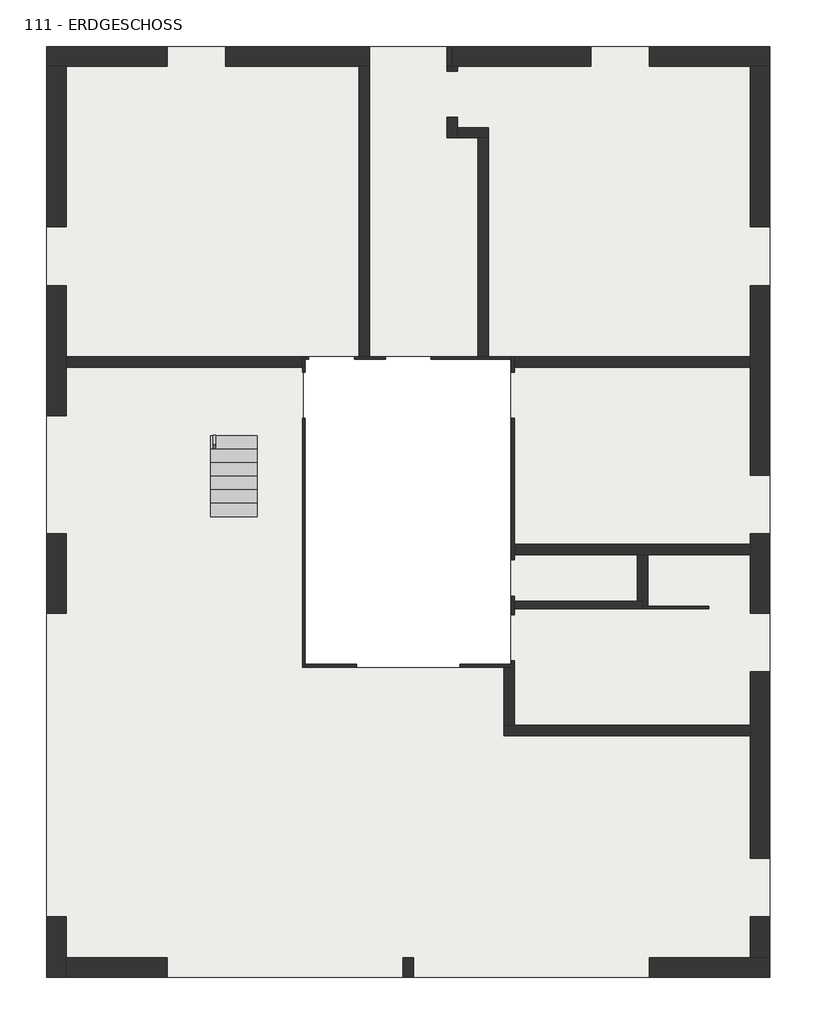
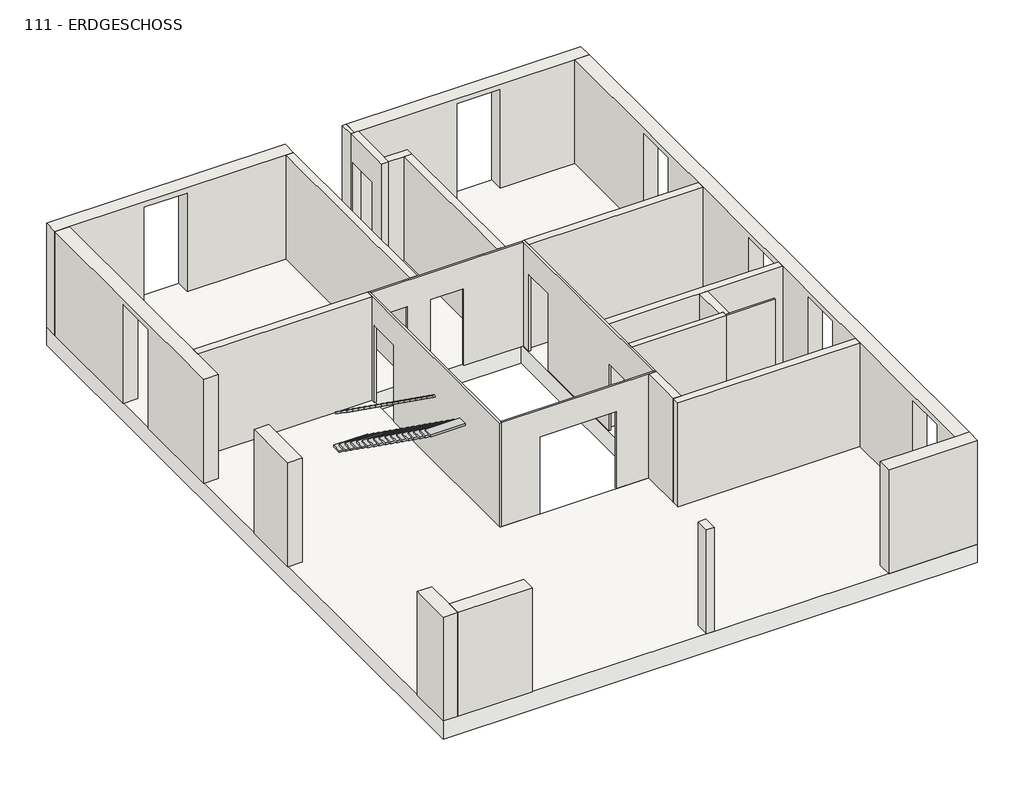
# One storey: 21 walls, 2 stairs, 1 slab.
"""IFC4 building model written with IfcOpenShell, lengths in millimetres."""

import ifcopenshell
import ifcopenshell.guid

model = None  # the IFC model being written
_history = None  # IfcOwnerHistory: only IFC2X3 demands one
_inside = {}  # id of a spatial element -> (the spatial element, [elements in it])
_under = {}  # id of a project, library or spatial element -> (it, [spatial elements below it])
_declared = {}  # id of a project -> (the project, [libraries it declares])
_typed = {}  # id of a type object -> (the type object, [elements of that type])
_made_of = {}  # id of a material, layer set ... -> (it, [elements and type objects made of it])


def new_model(schema):
    """Start an empty IFC model of exactly this schema.

    Asked for "IFC4X3", IfcOpenShell would pick the latest addendum, in which some entities
    have other attributes; the version numbers below select the first issue.
    IFC2X3 requires an IfcOwnerHistory on every rooted entity: one is made here for all.
    """
    global model, _history
    if schema == "IFC4X3":
        model = ifcopenshell.file(schema_version=(4, 3, 0, 0))
    else:
        model = ifcopenshell.file(schema=schema)
    _inside.clear()
    _under.clear()
    _declared.clear()
    _typed.clear()
    _made_of.clear()
    _history = None
    if model.schema == "IFC2X3":
        org = make("IfcOrganization", Name="unknown")
        user = make(
            "IfcPersonAndOrganization",
            ThePerson=make("IfcPerson", FamilyName="unknown"),
            TheOrganization=org,
        )
        app = make(
            "IfcApplication",
            ApplicationDeveloper=org,
            Version="unknown",
            ApplicationFullName="unknown",
            ApplicationIdentifier="unknown",
        )
        _history = make(
            "IfcOwnerHistory",
            OwningUser=user,
            OwningApplication=app,
            ChangeAction="ADDED",
            CreationDate=0,
        )
    return model


def make(cls, **values):
    """One entity of the class cls with the attributes given. An attribute that is None is left unset."""
    return model.create_entity(
        cls, **{name: value for name, value in values.items() if value is not None}
    )


def rooted(cls, **values):
    """An entity with a GlobalId (a new one), such as an element, a storey or a relation."""
    return make(cls, GlobalId=ifcopenshell.guid.new(), OwnerHistory=_history, **values)


def si_unit(unit_type, name, prefix=None):
    """IfcSIUnit, for example si_unit("LENGTHUNIT", "METRE", prefix="MILLI")."""
    return make("IfcSIUnit", UnitType=unit_type, Prefix=prefix, Name=name)


def assignment(units):
    """IfcUnitAssignment: the units of a project."""
    return None if units is None else make("IfcUnitAssignment", Units=units)


def point(xyz):
    """IfcCartesianPoint."""
    return None if xyz is None else make("IfcCartesianPoint", Coordinates=xyz)


def direction(xyz):
    """IfcDirection."""
    return None if xyz is None else make("IfcDirection", DirectionRatios=xyz)


def frame(location, z_axis=None, x_axis=None):
    """IfcAxis2Placement3D, a coordinate frame: its origin and axes. An axis left out is left unset."""
    return make(
        "IfcAxis2Placement3D",
        Location=point(location),
        Axis=direction(z_axis),
        RefDirection=direction(x_axis),
    )


def origin():
    """The frame at (0, 0, 0) with its axes left unset."""
    return frame((0.0, 0.0, 0.0))


def origin_with_axes():
    """The frame at (0, 0, 0) with the z axis (0, 0, 1) and the x axis (1, 0, 0) written out."""
    return frame((0.0, 0.0, 0.0), z_axis=(0.0, 0.0, 1.0), x_axis=(1.0, 0.0, 0.0))


def place(relative_to, where):
    """IfcLocalPlacement: puts the frame where relative to a parent placement (None: the world)."""
    return make(
        "IfcLocalPlacement", PlacementRelTo=relative_to, RelativePlacement=where
    )


def context(
    kind, dimensions, precision=None, world=None, true_north=None, identifier=None
):
    """IfcGeometricRepresentationContext, for example the 3D "Model" context."""
    return make(
        "IfcGeometricRepresentationContext",
        ContextIdentifier=identifier,
        ContextType=kind,
        CoordinateSpaceDimension=dimensions,
        Precision=precision,
        WorldCoordinateSystem=world,
        TrueNorth=true_north,
    )


def project(units=None, contexts=None):
    """IfcProject with its units and contexts."""
    return rooted(
        "IfcProject",
        Name="project",
        RepresentationContexts=contexts,
        UnitsInContext=assignment(units),
    )


def spatial(cls, under=None, at=None, **own):
    """A site, building, storey or space (cls), placed at a placement, below another one or the project."""
    s = rooted(cls, ObjectPlacement=at, **own)
    if under is not None:
        _under.setdefault(under.id(), (under, []))[1].append(s)
    return s


def polyline(points):
    """IfcPolyline through the points."""
    return make("IfcPolyline", Points=[point(p) for p in points])


def outline(outer, holes=None, kind="AREA"):
    """IfcArbitraryClosedProfileDef: a profile drawn as a closed curve; with holes, ...WithVoids."""
    if holes is None:
        return make("IfcArbitraryClosedProfileDef", ProfileType=kind, OuterCurve=outer)
    return make(
        "IfcArbitraryProfileDefWithVoids",
        ProfileType=kind,
        OuterCurve=outer,
        InnerCurves=holes,
    )


def extrude(swept, where, along, depth):
    """IfcExtrudedAreaSolid: the profile swept, set in the frame where, extruded along a direction by depth."""
    return make(
        "IfcExtrudedAreaSolid",
        SweptArea=swept,
        Position=where,
        ExtrudedDirection=direction(along),
        Depth=depth,
    )


def faces_of(points, faces, orient=None, outer=None):
    """IfcFace entities. A face is a list of loops; a loop is a list of indices into points, from 0.

    orient and outer hold one flag for each loop. By default every Orientation is true, the
    first loop of a face is its IfcFaceOuterBound and the others are IfcFaceBound.
    """
    made = []
    for i, loops in enumerate(faces):
        bounds = []
        for j, loop in enumerate(loops):
            is_outer = j == 0 if outer is None else outer[i][j]
            bounds.append(
                make(
                    "IfcFaceOuterBound" if is_outer else "IfcFaceBound",
                    Bound=make("IfcPolyLoop", Polygon=[points[k] for k in loop]),
                    Orientation=True if orient is None else orient[i][j],
                )
            )
        made.append(make("IfcFace", Bounds=bounds))
    return made


def faceted_brep(points, faces, orient=None, outer=None, voids=None):
    """IfcFacetedBrep: a solid bounded by flat faces; with voids (closed shells), ...WithVoids."""
    shared = [point(p) for p in points]
    hull = make("IfcClosedShell", CfsFaces=faces_of(shared, faces, orient, outer))
    if voids is None:
        return make("IfcFacetedBrep", Outer=hull)
    return make(
        "IfcFacetedBrepWithVoids",
        Outer=hull,
        Voids=[
            make(cls, CfsFaces=faces_of(shared, fs, o, b)) for cls, fs, o, b in voids
        ],
    )


def shape(context_of_items, identifier, shape_type, items):
    """IfcShapeRepresentation: the items that make up one representation, for example the "Body"."""
    return make(
        "IfcShapeRepresentation",
        ContextOfItems=context_of_items,
        RepresentationIdentifier=identifier,
        RepresentationType=shape_type,
        Items=items,
    )


def source(mapping_origin, context_of_items, identifier, shape_type, items):
    """IfcRepresentationMap: a shape defined once, which mapped items show again and again."""
    return make(
        "IfcRepresentationMap",
        MappingOrigin=mapping_origin,
        MappedRepresentation=shape(context_of_items, identifier, shape_type, items),
    )


def transform(
    local_origin,
    x_axis=None,
    y_axis=None,
    z_axis=None,
    scale=None,
    scale2=None,
    scale3=None,
    uniform=True,
):
    """IfcCartesianTransformationOperator3D, or its non-uniform kind. x_axis, y_axis, z_axis: its Axis1, 2, 3."""
    if uniform:
        return make(
            "IfcCartesianTransformationOperator3D",
            Axis1=direction(x_axis),
            Axis2=direction(y_axis),
            LocalOrigin=point(local_origin),
            Scale=scale,
            Axis3=direction(z_axis),
        )
    return make(
        "IfcCartesianTransformationOperator3DnonUniform",
        Axis1=direction(x_axis),
        Axis2=direction(y_axis),
        LocalOrigin=point(local_origin),
        Scale=scale,
        Axis3=direction(z_axis),
        Scale2=scale2,
        Scale3=scale3,
    )


def mapped(mapping_source, mapping_target):
    """IfcMappedItem: shows the shape of a source again, moved by a transform."""
    return make(
        "IfcMappedItem", MappingSource=mapping_source, MappingTarget=mapping_target
    )


def made_of(thing, what):
    """Note that an element or type object is made of a material, layer set ...; save() writes the relation."""
    if what is not None:
        _made_of.setdefault(what.id(), (what, []))[1].append(thing)
    return thing


def element(
    cls,
    number,
    at=None,
    inside=None,
    cuts=None,
    type_object=None,
    material=None,
    context=None,
    identifier="Body",
    shape_type=None,
    held_by="IfcProductDefinitionShape",
    body=None,
    shapes=None,
    **own,
):
    """One element of the class cls, such as IfcWall. Its Tag is "e" and its number.

    at: its placement. inside: the storey or other place that contains it. cuts: it is an
    opening in that element (IfcRelVoidsElement). A single representation is given by context,
    identifier, shape_type and body (its items); several are given by shapes. held_by: the class
    of the entity that holds the representations. save() writes the other relations.
    """
    e = rooted(cls, Tag="e%d" % number, ObjectPlacement=at, **own)
    if body is not None:
        shapes = [shape(context, identifier, shape_type, body)]
    if shapes is not None:
        e.Representation = make(held_by, Representations=shapes)
    if inside is not None:
        _inside.setdefault(inside.id(), (inside, []))[1].append(e)
    if cuts is not None:
        rooted(
            "IfcRelVoidsElement", RelatingBuildingElement=cuts, RelatedOpeningElement=e
        )
    if type_object is not None:
        _typed.setdefault(type_object.id(), (type_object, []))[1].append(e)
    return made_of(e, material)


def aggregate(whole, parts):
    """IfcRelAggregates: a whole, such as a stair, and the parts it consists of."""
    return rooted("IfcRelAggregates", RelatingObject=whole, RelatedObjects=parts)


def save(model, path):
    """Write the relations noted so far, then the file.

    IfcRelAggregates (storeys below a building ...), IfcRelContainedInSpatialStructure (elements
    in a storey), IfcRelDefinesByType, IfcRelAssociatesMaterial and IfcRelDeclares: one each for
    every whole, place, type object, material and project.
    """
    for whole, parts in _under.values():
        aggregate(whole, parts)
    for where, things in _inside.values():
        rooted(
            "IfcRelContainedInSpatialStructure",
            RelatedElements=things,
            RelatingStructure=where,
        )
    for kind, things in _typed.values():
        rooted("IfcRelDefinesByType", RelatedObjects=things, RelatingType=kind)
    for what, things in _made_of.values():
        rooted("IfcRelAssociatesMaterial", RelatedObjects=things, RelatingMaterial=what)
    for by, libraries in _declared.values():
        rooted("IfcRelDeclares", RelatingContext=by, RelatedDefinitions=libraries)
    model.write(path)


def slab_87d51967(model_context):
    return source(origin(), model_context, "Body", "SweptSolid", [
        extrude(outline(polyline([(15500.0, 1547.1380981), (1500.0, 1547.1380981), (1500.0, 19550.0), (15500.0, 19550.0), (15500.0, 1547.1380981)]), holes=[polyline([(10475.0, 13550.0), (6475.0, 13550.0), (6475.0, 7550.0), (10475.0, 7550.0), (10475.0, 13550.0)])]), frame((0.0, 0.0, -500.0), z_axis=(0.0, 0.0, 1.0), x_axis=(1.0, 0.0, 0.0)), (0.0, 0.0, 1.0), 500.0),
    ])


def stair_a78379cc(model_context):
    return source(origin(), model_context, "Body", "SweptSolid", [
        extrude(outline(polyline([(0.0, -319.1002977), (0.0, 0.0), (50.0, 0.0), (50.0, -319.1002977), (0.0, -319.1002977)])), frame((162072.7593015, 34520.3024209, 4178.947508), z_axis=(0.0, 0.5797550216229128, 0.8147908411997622), x_axis=(-1.0, 0.0, 0.0)), (0.0, 0.0, 1.0), 50.0),
        extrude(outline(polyline([(0.0, -319.1002977), (0.0, 0.0), (50.0, 0.0), (50.0, -319.1002977), (0.0, -319.1002977)])), frame((162072.7593015, 34780.3024209, 3993.947508), z_axis=(0.0, 0.5797550216228999, 0.8147908411997712), x_axis=(-1.0, 0.0, 0.0)), (0.0, 0.0, 1.0), 50.0),
        extrude(outline(polyline([(0.0, -319.1002977), (0.0, 0.0), (50.0, 0.0), (50.0, -319.1002977), (0.0, -319.1002977)])), frame((162072.7593015, 35040.3024209, 3808.947508), z_axis=(0.0, 0.5797550216229128, 0.8147908411997622), x_axis=(-1.0, 0.0, 0.0)), (0.0, 0.0, 1.0), 50.0),
        extrude(outline(polyline([(0.0, -319.1002977), (0.0, 0.0), (50.0, 0.0), (50.0, -319.1002977), (0.0, -319.1002977)])), frame((162072.7593015, 35300.3024209, 3623.947508), z_axis=(0.0, 0.5797550216229086, 0.8147908411997651), x_axis=(-1.0, 0.0, 0.0)), (0.0, 0.0, 1.0), 50.0),
        extrude(outline(polyline([(0.0, -319.1002977), (0.0, 0.0), (50.0, 0.0), (50.0, -319.1002977), (0.0, -319.1002977)])), frame((162072.7593015, 35560.3024209, 3438.947508), z_axis=(0.0, 0.5797550216229094, 0.8147908411997645), x_axis=(-1.0, 0.0, 0.0)), (0.0, 0.0, 1.0), 50.0),
        extrude(outline(polyline([(0.0, -319.1002977), (0.0, 0.0), (50.0, 0.0), (50.0, -319.1002977), (0.0, -319.1002977)])), frame((162072.7593015, 35820.3024209, 3253.947508), z_axis=(0.0, 0.5797550216229012, 0.8147908411997705), x_axis=(-1.0, 0.0, 0.0)), (0.0, 0.0, 1.0), 50.0),
        extrude(outline(polyline([(0.0, -319.1002977), (0.0, 0.0), (50.0, 0.0), (50.0, -319.1002977), (0.0, -319.1002977)])), frame((162072.7593015, 36080.3024209, 3068.947508), z_axis=(0.0, 0.5797550216229139, 0.8147908411997614), x_axis=(-1.0, 0.0, 0.0)), (0.0, 0.0, 1.0), 50.0),
        extrude(outline(polyline([(0.0, -319.1002977), (0.0, 0.0), (50.0, 0.0), (50.0, -319.1002977), (0.0, -319.1002977)])), frame((162072.7593015, 36340.3024209, 2883.947508), z_axis=(0.0, 0.579755021622915, 0.8147908411997605), x_axis=(-1.0, 0.0, 0.0)), (0.0, 0.0, 1.0), 50.0),
        extrude(outline(polyline([(0.0, -319.1002977), (0.0, 0.0), (50.0, 0.0), (50.0, -319.1002977), (0.0, -319.1002977)])), frame((162072.7593015, 36600.3024209, 2698.947508), z_axis=(0.0, 0.5797550216229116, 0.814790841199763), x_axis=(-1.0, 0.0, 0.0)), (0.0, 0.0, 1.0), 50.0),
        extrude(outline(polyline([(0.0, -319.1002977), (0.0, 0.0), (50.0, 0.0), (50.0, -319.1002977), (0.0, -319.1002977)])), frame((162072.7593015, 36860.3024209, 2513.947508), z_axis=(0.0, 0.5797550216228977, 0.8147908411997729), x_axis=(-1.0, 0.0, 0.0)), (0.0, 0.0, 1.0), 50.0),
        extrude(outline(polyline([(0.0, -319.1002977), (0.0, 0.0), (50.0, 0.0), (50.0, -319.1002977), (0.0, -319.1002977)])), frame((162072.7593015, 37120.3024209, 2328.947508), z_axis=(0.0, 0.5797550216229123, 0.8147908411997625), x_axis=(-1.0, 0.0, 0.0)), (0.0, 0.0, 1.0), 50.0),
        extrude(outline(polyline([(0.0, -319.1002977), (0.0, 0.0), (50.0, 0.0), (50.0, -319.1002977), (0.0, -319.1002977)])), frame((162072.7593015, 37380.3024209, 2143.947508), z_axis=(0.0, 0.5797550216229145, 0.814790841199761), x_axis=(-1.0, 0.0, 0.0)), (0.0, 0.0, 1.0), 50.0),
        extrude(outline(polyline([(0.0, -319.1002977), (0.0, 0.0), (50.0, 0.0), (50.0, -319.1002977), (0.0, -319.1002977)])), frame((162072.7593015, 37640.3024209, 1958.947508), z_axis=(0.0, 0.5797550216228994, 0.8147908411997717), x_axis=(-1.0, 0.0, 0.0)), (0.0, 0.0, 1.0), 50.0),
        extrude(outline(polyline([(0.0, -319.1002977), (0.0, 0.0), (50.0, 0.0), (50.0, -319.1002977), (0.0, -319.1002977)])), frame((162072.7593015, 37900.3024209, 1773.947508), z_axis=(0.0, 0.579755021622915, 0.8147908411997605), x_axis=(-1.0, 0.0, 0.0)), (0.0, 0.0, 1.0), 50.0),
        extrude(outline(polyline([(0.0, -319.1002977), (0.0, 0.0), (50.0, 0.0), (50.0, -319.1002977), (0.0, -319.1002977)])), frame((162072.7593015, 38160.3024209, 1588.947508), z_axis=(0.0, 0.5797550216229086, 0.8147908411997651), x_axis=(-1.0, 0.0, 0.0)), (0.0, 0.0, 1.0), 50.0),
        extrude(outline(polyline([(0.0, -319.1002977), (0.0, 0.0), (50.0, 0.0), (50.0, -319.1002977), (0.0, -319.1002977)])), frame((162072.7593015, 38420.3024209, 1403.947508), z_axis=(0.0, 0.5797550216229066, 0.8147908411997665), x_axis=(-1.0, 0.0, 0.0)), (0.0, 0.0, 1.0), 50.0),
        extrude(outline(polyline([(0.0, -319.1002977), (0.0, 0.0), (50.0, 0.0), (50.0, -319.1002977), (0.0, -319.1002977)])), frame((162072.7593015, 38680.3024209, 1218.947508), z_axis=(0.0, 0.5797550216228988, 0.8147908411997722), x_axis=(-1.0, 0.0, 0.0)), (0.0, 0.0, 1.0), 50.0),
        extrude(outline(polyline([(161972.7593015, 38694.7962965), (161972.7593015, 38954.7962965), (162872.7593015, 38954.7962965), (162872.7593015, 38694.7962965), (161972.7593015, 38694.7962965)])), frame((0.0, 0.0, 135.0), z_axis=(0.0, 0.0, 1.0), x_axis=(1.0, 0.0, 0.0)), (0.0, 0.0, 1.0), 50.0),
        extrude(outline(polyline([(161972.7593015, 38434.7962965), (161972.7593015, 38694.7962965), (162872.7593015, 38694.7962965), (162872.7593015, 38434.7962965), (161972.7593015, 38434.7962965)])), frame((0.0, 0.0, 320.0), z_axis=(0.0, 0.0, 1.0), x_axis=(1.0, 0.0, 0.0)), (0.0, 0.0, 1.0), 50.0),
        extrude(outline(polyline([(161972.7593015, 38174.7962965), (161972.7593015, 38434.7962965), (162872.7593015, 38434.7962965), (162872.7593015, 38174.7962965), (161972.7593015, 38174.7962965)])), frame((0.0, 0.0, 505.0), z_axis=(0.0, 0.0, 1.0), x_axis=(1.0, 0.0, 0.0)), (0.0, 0.0, 1.0), 50.0),
        extrude(outline(polyline([(161972.7593015, 37914.7962965), (161972.7593015, 38174.7962965), (162872.7593015, 38174.7962965), (162872.7593015, 37914.7962965), (161972.7593015, 37914.7962965)])), frame((0.0, 0.0, 690.0), z_axis=(0.0, 0.0, 1.0), x_axis=(1.0, 0.0, 0.0)), (0.0, 0.0, 1.0), 50.0),
        extrude(outline(polyline([(161972.7593015, 37654.7962965), (161972.7593015, 37914.7962965), (162872.7593015, 37914.7962965), (162872.7593015, 37654.7962965), (161972.7593015, 37654.7962965)])), frame((0.0, 0.0, 875.0), z_axis=(0.0, 0.0, 1.0), x_axis=(1.0, 0.0, 0.0)), (0.0, 0.0, 1.0), 50.0),
        extrude(outline(polyline([(161972.7593015, 37394.7962965), (161972.7593015, 37654.7962965), (162872.7593015, 37654.7962965), (162872.7593015, 37394.7962965), (161972.7593015, 37394.7962965)])), frame((0.0, 0.0, 1060.0), z_axis=(0.0, 0.0, 1.0), x_axis=(1.0, 0.0, 0.0)), (0.0, 0.0, 1.0), 50.0),
        extrude(outline(polyline([(161972.7593015, 37134.7962965), (161972.7593015, 37394.7962965), (162872.7593015, 37394.7962965), (162872.7593015, 37134.7962965), (161972.7593015, 37134.7962965)])), frame((0.0, 0.0, 1245.0), z_axis=(0.0, 0.0, 1.0), x_axis=(1.0, 0.0, 0.0)), (0.0, 0.0, 1.0), 50.0),
        extrude(outline(polyline([(161972.7593015, 36874.7962965), (161972.7593015, 37134.7962965), (162872.7593015, 37134.7962965), (162872.7593015, 36874.7962965), (161972.7593015, 36874.7962965)])), frame((0.0, 0.0, 1430.0), z_axis=(0.0, 0.0, 1.0), x_axis=(1.0, 0.0, 0.0)), (0.0, 0.0, 1.0), 50.0),
        extrude(outline(polyline([(161972.7593015, 36614.7962965), (161972.7593015, 36874.7962965), (162872.7593015, 36874.7962965), (162872.7593015, 36614.7962965), (161972.7593015, 36614.7962965)])), frame((0.0, 0.0, 1615.0), z_axis=(0.0, 0.0, 1.0), x_axis=(1.0, 0.0, 0.0)), (0.0, 0.0, 1.0), 50.0),
        extrude(outline(polyline([(161972.7593015, 36354.7962965), (161972.7593015, 36614.7962965), (162872.7593015, 36614.7962965), (162872.7593015, 36354.7962965), (161972.7593015, 36354.7962965)])), frame((0.0, 0.0, 1800.0), z_axis=(0.0, 0.0, 1.0), x_axis=(1.0, 0.0, 0.0)), (0.0, 0.0, 1.0), 50.0),
        extrude(outline(polyline([(161972.7593015, 36094.7962965), (161972.7593015, 36354.7962965), (162872.7593015, 36354.7962965), (162872.7593015, 36094.7962965), (161972.7593015, 36094.7962965)])), frame((0.0, 0.0, 1985.0), z_axis=(0.0, 0.0, 1.0), x_axis=(1.0, 0.0, 0.0)), (0.0, 0.0, 1.0), 50.0),
        extrude(outline(polyline([(161972.7593015, 35834.7962965), (161972.7593015, 36094.7962965), (162872.7593015, 36094.7962965), (162872.7593015, 35834.7962965), (161972.7593015, 35834.7962965)])), frame((0.0, 0.0, 2170.0), z_axis=(0.0, 0.0, 1.0), x_axis=(1.0, 0.0, 0.0)), (0.0, 0.0, 1.0), 50.0),
        extrude(outline(polyline([(161972.7593015, 35574.7962965), (161972.7593015, 35834.7962965), (162872.7593015, 35834.7962965), (162872.7593015, 35574.7962965), (161972.7593015, 35574.7962965)])), frame((0.0, 0.0, 2355.0), z_axis=(0.0, 0.0, 1.0), x_axis=(1.0, 0.0, 0.0)), (0.0, 0.0, 1.0), 50.0),
        extrude(outline(polyline([(161972.7593015, 35314.7962965), (161972.7593015, 35574.7962965), (162872.7593015, 35574.7962965), (162872.7593015, 35314.7962965), (161972.7593015, 35314.7962965)])), frame((0.0, 0.0, 2540.0), z_axis=(0.0, 0.0, 1.0), x_axis=(1.0, 0.0, 0.0)), (0.0, 0.0, 1.0), 50.0),
        extrude(outline(polyline([(161972.7593015, 35054.7962965), (161972.7593015, 35314.7962965), (162872.7593015, 35314.7962965), (162872.7593015, 35054.7962965), (161972.7593015, 35054.7962965)])), frame((0.0, 0.0, 2725.0), z_axis=(0.0, 0.0, 1.0), x_axis=(1.0, 0.0, 0.0)), (0.0, 0.0, 1.0), 50.0),
        extrude(outline(polyline([(161972.7593015, 34794.7962965), (161972.7593015, 35054.7962965), (162872.7593015, 35054.7962965), (162872.7593015, 34794.7962965), (161972.7593015, 34794.7962965)])), frame((0.0, 0.0, 2910.0), z_axis=(0.0, 0.0, 1.0), x_axis=(1.0, 0.0, 0.0)), (0.0, 0.0, 1.0), 50.0),
        extrude(outline(polyline([(161972.7593015, 34534.7962965), (161972.7593015, 34794.7962965), (162872.7593015, 34794.7962965), (162872.7593015, 34534.7962965), (161972.7593015, 34534.7962965)])), frame((0.0, 0.0, 3095.0), z_axis=(0.0, 0.0, 1.0), x_axis=(1.0, 0.0, 0.0)), (0.0, 0.0, 1.0), 50.0),
    ])


def stair_667f7fc2(model_context):
    return source(origin(), model_context, "Body", "SweptSolid", [
        extrude(outline(polyline([(0.0, -319.1002977), (0.0, 0.0), (50.0, 0.0), (50.0, -319.1002977), (0.0, -319.1002977)])), frame((162072.7593015, 34520.3024209, 4178.947508), z_axis=(0.0, 0.5797550216229128, 0.8147908411997622), x_axis=(-1.0, 0.0, 0.0)), (0.0, 0.0, 1.0), 50.0),
        extrude(outline(polyline([(0.0, -319.1002977), (0.0, 0.0), (50.0, 0.0), (50.0, -319.1002977), (0.0, -319.1002977)])), frame((162072.7593015, 34780.3024209, 3993.947508), z_axis=(0.0, 0.5797550216229022, 0.8147908411997696), x_axis=(-1.0, 0.0, 0.0)), (0.0, 0.0, 1.0), 50.0),
        extrude(outline(polyline([(0.0, -319.1002977), (0.0, 0.0), (50.0, 0.0), (50.0, -319.1002977), (0.0, -319.1002977)])), frame((162072.7593015, 35040.3024209, 3808.947508), z_axis=(0.0, 0.5797550216229116, 0.814790841199763), x_axis=(-1.0, 0.0, 0.0)), (0.0, 0.0, 1.0), 50.0),
        extrude(outline(polyline([(0.0, -319.1002977), (0.0, 0.0), (50.0, 0.0), (50.0, -319.1002977), (0.0, -319.1002977)])), frame((162072.7593015, 35300.3024209, 3623.947508), z_axis=(0.0, 0.5797550216229086, 0.8147908411997651), x_axis=(-1.0, 0.0, 0.0)), (0.0, 0.0, 1.0), 50.0),
        extrude(outline(polyline([(0.0, -319.1002977), (0.0, 0.0), (50.0, 0.0), (50.0, -319.1002977), (0.0, -319.1002977)])), frame((162072.7593015, 35560.3024209, 3438.947508), z_axis=(0.0, 0.5797550216229094, 0.8147908411997645), x_axis=(-1.0, 0.0, 0.0)), (0.0, 0.0, 1.0), 50.0),
        extrude(outline(polyline([(0.0, -319.1002977), (0.0, 0.0), (50.0, 0.0), (50.0, -319.1002977), (0.0, -319.1002977)])), frame((162072.7593015, 35820.3024209, 3253.947508), z_axis=(0.0, 0.5797550216228999, 0.8147908411997712), x_axis=(-1.0, 0.0, 0.0)), (0.0, 0.0, 1.0), 50.0),
        extrude(outline(polyline([(0.0, -319.1002977), (0.0, 0.0), (50.0, 0.0), (50.0, -319.1002977), (0.0, -319.1002977)])), frame((162072.7593015, 36080.3024209, 3068.947508), z_axis=(0.0, 0.579755021622915, 0.8147908411997605), x_axis=(-1.0, 0.0, 0.0)), (0.0, 0.0, 1.0), 50.0),
        extrude(outline(polyline([(0.0, -319.1002977), (0.0, 0.0), (50.0, 0.0), (50.0, -319.1002977), (0.0, -319.1002977)])), frame((162072.7593015, 36340.3024209, 2883.947508), z_axis=(0.0, 0.5797550216229139, 0.8147908411997614), x_axis=(-1.0, 0.0, 0.0)), (0.0, 0.0, 1.0), 50.0),
        extrude(outline(polyline([(0.0, -319.1002977), (0.0, 0.0), (50.0, 0.0), (50.0, -319.1002977), (0.0, -319.1002977)])), frame((162072.7593015, 36600.3024209, 2698.947508), z_axis=(0.0, 0.5797550216229128, 0.8147908411997622), x_axis=(-1.0, 0.0, 0.0)), (0.0, 0.0, 1.0), 50.0),
        extrude(outline(polyline([(0.0, -319.1002977), (0.0, 0.0), (50.0, 0.0), (50.0, -319.1002977), (0.0, -319.1002977)])), frame((162072.7593015, 36860.3024209, 2513.947508), z_axis=(0.0, 0.5797550216228966, 0.8147908411997736), x_axis=(-1.0, 0.0, 0.0)), (0.0, 0.0, 1.0), 50.0),
        extrude(outline(polyline([(0.0, -319.1002977), (0.0, 0.0), (50.0, 0.0), (50.0, -319.1002977), (0.0, -319.1002977)])), frame((162072.7593015, 37120.3024209, 2328.947508), z_axis=(0.0, 0.5797550216229123, 0.8147908411997625), x_axis=(-1.0, 0.0, 0.0)), (0.0, 0.0, 1.0), 50.0),
        extrude(outline(polyline([(0.0, -319.1002977), (0.0, 0.0), (50.0, 0.0), (50.0, -319.1002977), (0.0, -319.1002977)])), frame((162072.7593015, 37380.3024209, 2143.947508), z_axis=(0.0, 0.5797550216229139, 0.8147908411997614), x_axis=(-1.0, 0.0, 0.0)), (0.0, 0.0, 1.0), 50.0),
        extrude(outline(polyline([(0.0, -319.1002977), (0.0, 0.0), (50.0, 0.0), (50.0, -319.1002977), (0.0, -319.1002977)])), frame((162072.7593015, 37640.3024209, 1958.947508), z_axis=(0.0, 0.5797550216228999, 0.8147908411997712), x_axis=(-1.0, 0.0, 0.0)), (0.0, 0.0, 1.0), 50.0),
        extrude(outline(polyline([(0.0, -319.1002977), (0.0, 0.0), (50.0, 0.0), (50.0, -319.1002977), (0.0, -319.1002977)])), frame((162072.7593015, 37900.3024209, 1773.947508), z_axis=(0.0, 0.579755021622915, 0.8147908411997605), x_axis=(-1.0, 0.0, 0.0)), (0.0, 0.0, 1.0), 50.0),
        extrude(outline(polyline([(0.0, -319.1002977), (0.0, 0.0), (50.0, 0.0), (50.0, -319.1002977), (0.0, -319.1002977)])), frame((162072.7593015, 38160.3024209, 1588.947508), z_axis=(0.0, 0.579755021622908, 0.8147908411997654), x_axis=(-1.0, 0.0, 0.0)), (0.0, 0.0, 1.0), 50.0),
        extrude(outline(polyline([(0.0, -319.1002977), (0.0, 0.0), (50.0, 0.0), (50.0, -319.1002977), (0.0, -319.1002977)])), frame((162072.7593015, 38420.3024209, 1403.947508), z_axis=(0.0, 0.5797550216229066, 0.8147908411997665), x_axis=(-1.0, 0.0, 0.0)), (0.0, 0.0, 1.0), 50.0),
        extrude(outline(polyline([(0.0, -319.1002977), (0.0, 0.0), (50.0, 0.0), (50.0, -319.1002977), (0.0, -319.1002977)])), frame((162072.7593015, 38680.3024209, 1218.947508), z_axis=(0.0, 0.5797550216228985, 0.8147908411997723), x_axis=(-1.0, 0.0, 0.0)), (0.0, 0.0, 1.0), 50.0),
        extrude(outline(polyline([(161972.7593015, 38694.7962965), (161972.7593015, 38954.7962965), (162872.7593015, 38954.7962965), (162872.7593015, 38694.7962965), (161972.7593015, 38694.7962965)])), frame((0.0, 0.0, 135.0), z_axis=(0.0, 0.0, 1.0), x_axis=(1.0, 0.0, 0.0)), (0.0, 0.0, 1.0), 50.0),
        extrude(outline(polyline([(161972.7593015, 38434.7962965), (161972.7593015, 38694.7962965), (162872.7593015, 38694.7962965), (162872.7593015, 38434.7962965), (161972.7593015, 38434.7962965)])), frame((0.0, 0.0, 320.0), z_axis=(0.0, 0.0, 1.0), x_axis=(1.0, 0.0, 0.0)), (0.0, 0.0, 1.0), 50.0),
        extrude(outline(polyline([(161972.7593015, 38174.7962965), (161972.7593015, 38434.7962965), (162872.7593015, 38434.7962965), (162872.7593015, 38174.7962965), (161972.7593015, 38174.7962965)])), frame((0.0, 0.0, 505.0), z_axis=(0.0, 0.0, 1.0), x_axis=(1.0, 0.0, 0.0)), (0.0, 0.0, 1.0), 50.0),
        extrude(outline(polyline([(161972.7593015, 37914.7962965), (161972.7593015, 38174.7962965), (162872.7593015, 38174.7962965), (162872.7593015, 37914.7962965), (161972.7593015, 37914.7962965)])), frame((0.0, 0.0, 690.0), z_axis=(0.0, 0.0, 1.0), x_axis=(1.0, 0.0, 0.0)), (0.0, 0.0, 1.0), 50.0),
        extrude(outline(polyline([(161972.7593015, 37654.7962965), (161972.7593015, 37914.7962965), (162872.7593015, 37914.7962965), (162872.7593015, 37654.7962965), (161972.7593015, 37654.7962965)])), frame((0.0, 0.0, 875.0), z_axis=(0.0, 0.0, 1.0), x_axis=(1.0, 0.0, 0.0)), (0.0, 0.0, 1.0), 50.0),
        extrude(outline(polyline([(161972.7593015, 37394.7962965), (161972.7593015, 37654.7962965), (162872.7593015, 37654.7962965), (162872.7593015, 37394.7962965), (161972.7593015, 37394.7962965)])), frame((0.0, 0.0, 1060.0), z_axis=(0.0, 0.0, 1.0), x_axis=(1.0, 0.0, 0.0)), (0.0, 0.0, 1.0), 50.0),
        extrude(outline(polyline([(161972.7593015, 37134.7962965), (161972.7593015, 37394.7962965), (162872.7593015, 37394.7962965), (162872.7593015, 37134.7962965), (161972.7593015, 37134.7962965)])), frame((0.0, 0.0, 1245.0), z_axis=(0.0, 0.0, 1.0), x_axis=(1.0, 0.0, 0.0)), (0.0, 0.0, 1.0), 50.0),
        extrude(outline(polyline([(161972.7593015, 36874.7962965), (161972.7593015, 37134.7962965), (162872.7593015, 37134.7962965), (162872.7593015, 36874.7962965), (161972.7593015, 36874.7962965)])), frame((0.0, 0.0, 1430.0), z_axis=(0.0, 0.0, 1.0), x_axis=(1.0, 0.0, 0.0)), (0.0, 0.0, 1.0), 50.0),
        extrude(outline(polyline([(161972.7593015, 36614.7962965), (161972.7593015, 36874.7962965), (162872.7593015, 36874.7962965), (162872.7593015, 36614.7962965), (161972.7593015, 36614.7962965)])), frame((0.0, 0.0, 1615.0), z_axis=(0.0, 0.0, 1.0), x_axis=(1.0, 0.0, 0.0)), (0.0, 0.0, 1.0), 50.0),
        extrude(outline(polyline([(161972.7593015, 36354.7962965), (161972.7593015, 36614.7962965), (162872.7593015, 36614.7962965), (162872.7593015, 36354.7962965), (161972.7593015, 36354.7962965)])), frame((0.0, 0.0, 1800.0), z_axis=(0.0, 0.0, 1.0), x_axis=(1.0, 0.0, 0.0)), (0.0, 0.0, 1.0), 50.0),
        extrude(outline(polyline([(161972.7593015, 36094.7962965), (161972.7593015, 36354.7962965), (162872.7593015, 36354.7962965), (162872.7593015, 36094.7962965), (161972.7593015, 36094.7962965)])), frame((0.0, 0.0, 1985.0), z_axis=(0.0, 0.0, 1.0), x_axis=(1.0, 0.0, 0.0)), (0.0, 0.0, 1.0), 50.0),
        extrude(outline(polyline([(161972.7593015, 35834.7962965), (161972.7593015, 36094.7962965), (162872.7593015, 36094.7962965), (162872.7593015, 35834.7962965), (161972.7593015, 35834.7962965)])), frame((0.0, 0.0, 2170.0), z_axis=(0.0, 0.0, 1.0), x_axis=(1.0, 0.0, 0.0)), (0.0, 0.0, 1.0), 50.0),
        extrude(outline(polyline([(161972.7593015, 35574.7962965), (161972.7593015, 35834.7962965), (162872.7593015, 35834.7962965), (162872.7593015, 35574.7962965), (161972.7593015, 35574.7962965)])), frame((0.0, 0.0, 2355.0), z_axis=(0.0, 0.0, 1.0), x_axis=(1.0, 0.0, 0.0)), (0.0, 0.0, 1.0), 50.0),
        extrude(outline(polyline([(161972.7593015, 35314.7962965), (161972.7593015, 35574.7962965), (162872.7593015, 35574.7962965), (162872.7593015, 35314.7962965), (161972.7593015, 35314.7962965)])), frame((0.0, 0.0, 2540.0), z_axis=(0.0, 0.0, 1.0), x_axis=(1.0, 0.0, 0.0)), (0.0, 0.0, 1.0), 50.0),
        extrude(outline(polyline([(161972.7593015, 35054.7962965), (161972.7593015, 35314.7962965), (162872.7593015, 35314.7962965), (162872.7593015, 35054.7962965), (161972.7593015, 35054.7962965)])), frame((0.0, 0.0, 2725.0), z_axis=(0.0, 0.0, 1.0), x_axis=(1.0, 0.0, 0.0)), (0.0, 0.0, 1.0), 50.0),
        extrude(outline(polyline([(161972.7593015, 34794.7962965), (161972.7593015, 35054.7962965), (162872.7593015, 35054.7962965), (162872.7593015, 34794.7962965), (161972.7593015, 34794.7962965)])), frame((0.0, 0.0, 2910.0), z_axis=(0.0, 0.0, 1.0), x_axis=(1.0, 0.0, 0.0)), (0.0, 0.0, 1.0), 50.0),
        extrude(outline(polyline([(161972.7593015, 34534.7962965), (161972.7593015, 34794.7962965), (162872.7593015, 34794.7962965), (162872.7593015, 34534.7962965), (161972.7593015, 34534.7962965)])), frame((0.0, 0.0, 3095.0), z_axis=(0.0, 0.0, 1.0), x_axis=(1.0, 0.0, 0.0)), (0.0, 0.0, 1.0), 50.0),
    ])


model = new_model("IFC4")

# Units and contexts
model_context = context("Model", 3, world=origin())
ifc_project = project(units=[si_unit("LENGTHUNIT", "METRE", prefix="MILLI")], contexts=[model_context])

# Site, building, storey
site = spatial("IfcSite", under=ifc_project)
building = spatial("IfcBuilding", under=site)
storey = spatial("IfcBuildingStorey", under=building, Name="111 - ERDGESCHOSS", Elevation=0.0)

# Slab
placement = place(None, origin())
slab_shape = slab_87d51967(model_context)
element("IfcSlab", 1, ObjectType="Holzdecke : Holzdecke", at=placement, inside=storey, context=model_context, shape_type="MappedRepresentation", body=[
    mapped(slab_shape, transform((0.0, 0.0, 0.0), x_axis=(1.0, 0.0, 0.0), y_axis=(0.0, 1.0, 0.0), z_axis=(0.0, 0.0, 1.0))),
])

# Stairs
stair_shape = stair_a78379cc(model_context)
element("IfcStair", 2, ObjectType="  :  ", at=placement, inside=storey, context=model_context, shape_type="MappedRepresentation", body=[
    mapped(stair_shape, transform((-157297.7593015, -26934.7962965, 0.0), x_axis=(1.0, 0.0, 0.0), y_axis=(0.0, 1.0, 0.0), z_axis=(0.0, 0.0, 1.0))),
])
stair_2_shape = stair_667f7fc2(model_context)
element("IfcStair", 3, ObjectType="  92587 :   92587", at=placement, inside=storey, context=model_context, shape_type="MappedRepresentation", body=[
    mapped(stair_2_shape, transform((-157297.7593015, -26934.7962965, 0.0), x_axis=(1.0, 0.0, 0.0), y_axis=(0.0, 1.0, 0.0), z_axis=(0.0, 0.0, 1.0))),
])

# Walls
element("IfcWall", 4, ObjectType="Holzwand:1129", at=placement, inside=storey, context=model_context, shape_type="SweptSolid", body=[
    extrude(outline(polyline([(7750.0, 19170.0), (7750.0, 13550.0), (7550.0, 13550.0), (7550.0, 19170.0), (7750.0, 19170.0)])), origin_with_axes(), (0.0, 0.0, 1.0), 2880.0),
])
element("IfcWall", 5, ObjectType="Holzwand:1130", at=placement, inside=storey, context=model_context, shape_type="SweptSolid", body=[
    extrude(outline(polyline([(6450.0, 13350.0), (1880.0, 13350.0), (1880.0, 13550.0), (6450.0, 13550.0), (6450.0, 13350.0)])), origin_with_axes(), (0.0, 0.0, 1.0), 2880.0),
])
element("IfcWall", 6, ObjectType="Holzwand:1131", at=placement, inside=storey, context=model_context, shape_type="Brep", body=[
    faceted_brep([(10050.0, 17981.8742346, 0.0), (9450.0, 17981.8742346, 0.0), (9450.0, 17981.8742346, 2880.0), (10050.0, 17981.8742346, 2880.0), (10050.0, 17781.8742346, 0.0), (10050.0, 17781.8742346, 2880.0), (9850.0, 17781.8742346, 2880.0), (9450.0, 17781.8742346, 2880.0), (9450.0, 17781.8742346, 0.0), (9850.0, 17781.8742346, 0.0)], [[[0, 1, 2, 3]], [[4, 5, 6, 7, 8, 9]], [[1, 0, 4, 9, 8]], [[3, 2, 7, 6, 5]], [[0, 3, 5, 4]], [[2, 1, 8, 7]]]),
])
element("IfcWall", 7, ObjectType="Holzwand:1132", at=placement, inside=storey, context=model_context, shape_type="Brep", body=[
    faceted_brep([(9450.0, 19170.0, 2880.0), (9450.0, 17981.8742346, 2880.0), (9450.0, 17781.8742346, 2880.0), (9450.0, 17781.8742346, 0.0), (9450.0, 17981.8742346, 0.0), (9450.0, 18184.2114284, 0.0), (9450.0, 18184.2114284, 2135.0), (9450.0, 19069.2114284, 2135.0), (9450.0, 19069.2114284, 0.0), (9450.0, 19170.0, 0.0), (9250.0, 17781.8742346, 2880.0), (9250.0, 19170.0, 2880.0), (9250.0, 19170.0, 0.0), (9250.0, 19069.2114284, 0.0), (9250.0, 19069.2114284, 2135.0), (9250.0, 18184.2114284, 2135.0), (9250.0, 18184.2114284, 0.0), (9250.0, 17781.8742346, 0.0)], [[[0, 1, 2, 3, 4, 5, 6, 7, 8, 9]], [[10, 11, 12, 13, 14, 15, 16, 17]], [[3, 17, 16, 5, 4]], [[12, 9, 8, 13]], [[2, 1, 0, 11, 10]], [[15, 6, 5, 16]], [[6, 15, 14, 7]], [[7, 14, 13, 8]], [[3, 2, 10, 17]], [[0, 9, 12, 11]]]),
])
element("IfcWall", 8, ObjectType="Holzwand:1133", at=placement, inside=storey, context=model_context, shape_type="SweptSolid", body=[
    extrude(outline(polyline([(10050.0, 17781.8742346), (10050.0, 13550.0), (9850.0, 13550.0), (9850.0, 17781.8742346), (10050.0, 17781.8742346)])), origin_with_axes(), (0.0, 0.0, 1.0), 2880.0),
])
element("IfcWall", 9, ObjectType="Holzwand:1134", at=placement, inside=storey, context=model_context, shape_type="SweptSolid", body=[
    extrude(outline(polyline([(15120.0, 13350.0), (10550.0, 13350.0), (10550.0, 13550.0), (15120.0, 13550.0), (15120.0, 13350.0)])), origin_with_axes(), (0.0, 0.0, 1.0), 2880.0),
])
element("IfcWall", 10, ObjectType="Holzwand:1136", at=placement, inside=storey, context=model_context, shape_type="Brep", body=[
    faceted_brep([(15120.0, 6425.0, 0.0), (10550.0, 6425.0, 0.0), (10350.0, 6425.0, 0.0), (10350.0, 6425.0, 2880.0), (10550.0, 6425.0, 2880.0), (15120.0, 6425.0, 2880.0), (15120.0, 6225.0, 0.0), (15120.0, 6225.0, 2880.0), (10350.0, 6225.0, 2880.0), (10350.0, 6225.0, 0.0)], [[[0, 1, 2, 3, 4, 5]], [[6, 7, 8, 9]], [[2, 1, 0, 6, 9]], [[5, 4, 3, 8, 7]], [[0, 5, 7, 6]], [[3, 2, 9, 8]]]),
])
element("IfcWall", 11, ObjectType="Holzwand:1137", at=placement, inside=storey, context=model_context, shape_type="SweptSolid", body=[
    extrude(outline(polyline([(10550.0, 9925.0), (15120.0, 9925.0), (15120.0, 9725.0), (10550.0, 9725.0), (10550.0, 9925.0)])), origin_with_axes(), (0.0, 0.0, 1.0), 2880.0),
])
element("IfcWall", 12, ObjectType="Holzwand:1139", at=placement, inside=storey, context=model_context, shape_type="SweptSolid", body=[
    extrude(outline(polyline([(10350.0, 6425.0), (10350.0, 7550.0), (10550.0, 7550.0), (10550.0, 6425.0), (10350.0, 6425.0)])), origin_with_axes(), (0.0, 0.0, 1.0), 2880.0),
])
element("IfcWall", 13, ObjectType="Holzwand:1143", at=placement, inside=storey, context=model_context, shape_type="Brep", body=[
    faceted_brep([(13035.0, 8825.0, 0.0), (12935.0, 8825.0, 0.0), (10550.0, 8825.0, 0.0), (10550.0, 8825.0, 2880.0), (12935.0, 8825.0, 2880.0), (13035.0, 8825.0, 2880.0), (13035.0, 8675.0, 0.0), (13035.0, 8675.0, 2880.0), (10550.0, 8675.0, 2880.0), (10550.0, 8675.0, 0.0), (13035.0, 8725.0, 0.0), (13035.0, 8725.0, 2880.0)], [[[0, 1, 2, 3, 4, 5]], [[6, 7, 8, 9]], [[2, 1, 0, 10, 6, 9]], [[3, 2, 9, 8]], [[5, 4, 3, 8, 7, 11]], [[0, 5, 11, 7, 6, 10]]]),
])
element("IfcWall", 14, ObjectType="Holzwand:1144", at=placement, inside=storey, context=model_context, shape_type="Brep", body=[
    faceted_brep([(13035.0, 8675.0, 0.0), (14320.0, 8675.0, 0.0), (14320.0, 8675.0, 2880.0), (13035.0, 8675.0, 2880.0), (13035.0, 8725.0, 0.0), (13035.0, 8725.0, 2880.0), (13135.0, 8725.0, 2880.0), (14320.0, 8725.0, 2880.0), (14320.0, 8725.0, 0.0), (13135.0, 8725.0, 0.0)], [[[0, 1, 2, 3]], [[4, 5, 6, 7, 8, 9]], [[1, 0, 4, 9, 8]], [[2, 1, 8, 7]], [[3, 2, 7, 6, 5]], [[0, 3, 5, 4]]]),
])
element("IfcWall", 15, ObjectType="Holzwand:1145", at=placement, inside=storey, context=model_context, shape_type="SweptSolid", body=[
    extrude(outline(polyline([(12935.0, 8825.0), (12935.0, 9725.0), (13135.0, 9725.0), (13135.0, 8725.0), (13035.0, 8725.0), (13035.0, 8825.0), (12935.0, 8825.0)])), origin_with_axes(), (0.0, 0.0, 1.0), 2880.0),
])
element("IfcWall", 16, ObjectType=" :1146", at=placement, inside=storey, context=model_context, shape_type="Brep", body=[
    faceted_brep([(6500.0, 13550.0, 2880.0), (6500.0, 13500.0, 2880.0), (6500.0, 7600.0, 2880.0), (6500.0, 7550.0, 2880.0), (6500.0, 7550.0, 0.0), (6500.0, 7600.0, 0.0), (6500.0, 12363.6489699, 0.0), (6500.0, 12363.6489699, 2135.0), (6500.0, 13248.6489699, 2135.0), (6500.0, 13248.6489699, 0.0), (6500.0, 13500.0, 0.0), (6500.0, 13550.0, 0.0), (6450.0, 7550.0, 2880.0), (6450.0, 13550.0, 2880.0), (6450.0, 13550.0, 0.0), (6450.0, 13248.6489699, 0.0), (6450.0, 13248.6489699, 2135.0), (6450.0, 12363.6489699, 2135.0), (6450.0, 12363.6489699, 0.0), (6450.0, 7550.0, 0.0)], [[[0, 1, 2, 3, 4, 5, 6, 7, 8, 9, 10, 11]], [[12, 13, 14, 15, 16, 17, 18, 19]], [[14, 11, 10, 9, 15]], [[4, 19, 18, 6, 5]], [[3, 2, 1, 0, 13, 12]], [[8, 16, 15, 9]], [[16, 8, 7, 17]], [[17, 7, 6, 18]], [[0, 11, 14, 13]], [[4, 3, 12, 19]]]),
])
element("IfcWall", 17, ObjectType=" :1147", at=placement, inside=storey, context=model_context, shape_type="SweptSolid", body=[
    extrude(outline(polyline([(2880.0, 10500.0), (2880.0, 6500.0), (0.0, 6500.0), (0.0, 6572.8375746), (2150.0, 6572.8375746), (2150.0, 7457.8375746), (0.0, 7457.8375746), (0.0, 8057.5), (2135.0, 8057.5), (2135.0, 8942.5), (0.0, 8942.5), (0.0, 10500.0), (2880.0, 10500.0)])), frame((0.0, 13500.0, 0.0), z_axis=(0.0, 1.0, 0.0), x_axis=(0.0, 0.0, 1.0)), (0.0, 0.0, 1.0), 50.0),
])
element("IfcWall", 18, ObjectType=" :1148", at=placement, inside=storey, context=model_context, shape_type="Brep", body=[
    faceted_brep([(6500.0, 7600.0, 2880.0), (10500.0, 7600.0, 2880.0), (10550.0, 7600.0, 2880.0), (10550.0, 7600.0, 0.0), (10500.0, 7600.0, 0.0), (9500.0, 7600.0, 0.0), (9500.0, 7600.0, 2135.0), (7500.0, 7600.0, 2135.0), (7500.0, 7600.0, 0.0), (6500.0, 7600.0, 0.0), (10550.0, 7550.0, 2880.0), (6500.0, 7550.0, 2880.0), (6500.0, 7550.0, 0.0), (7500.0, 7550.0, 0.0), (7500.0, 7550.0, 2135.0), (9500.0, 7550.0, 2135.0), (9500.0, 7550.0, 0.0), (10550.0, 7550.0, 0.0)], [[[0, 1, 2, 3, 4, 5, 6, 7, 8, 9]], [[10, 11, 12, 13, 14, 15, 16, 17]], [[3, 17, 16, 5, 4]], [[12, 9, 8, 13]], [[2, 1, 0, 11, 10]], [[7, 14, 13, 8]], [[14, 7, 6, 15]], [[15, 6, 5, 16]], [[3, 2, 10, 17]], [[0, 9, 12, 11]]]),
])
element("IfcWall", 19, ObjectType=" :1149", at=placement, inside=storey, context=model_context, shape_type="Brep", body=[
    faceted_brep([(10500.0, 7600.0, 2880.0), (10500.0, 13500.0, 2880.0), (10500.0, 13550.0, 2880.0), (10500.0, 13550.0, 0.0), (10500.0, 13500.0, 0.0), (10500.0, 13248.6489699, 0.0), (10500.0, 13248.6489699, 2135.0), (10500.0, 12363.6489699, 2135.0), (10500.0, 12363.6489699, 0.0), (10500.0, 9621.2509729, 0.0), (10500.0, 9621.2509729, 1860.0), (10500.0, 8921.2509729, 1860.0), (10500.0, 8921.2509729, 0.0), (10500.0, 8561.3454038, 0.0), (10500.0, 8561.3454038, 1860.0), (10500.0, 7676.3454038, 1860.0), (10500.0, 7676.3454038, 0.0), (10500.0, 7600.0, 0.0), (10550.0, 13550.0, 2880.0), (10550.0, 7600.0, 2880.0), (10550.0, 7600.0, 0.0), (10550.0, 7676.3454038, 0.0), (10550.0, 7676.3454038, 1860.0), (10550.0, 8561.3454038, 1860.0), (10550.0, 8561.3454038, 0.0), (10550.0, 8921.2509729, 0.0), (10550.0, 8921.2509729, 1860.0), (10550.0, 9621.2509729, 1860.0), (10550.0, 9621.2509729, 0.0), (10550.0, 12363.6489699, 0.0), (10550.0, 12363.6489699, 2135.0), (10550.0, 13248.6489699, 2135.0), (10550.0, 13248.6489699, 0.0), (10550.0, 13550.0, 0.0)], [[[0, 1, 2, 3, 4, 5, 6, 7, 8, 9, 10, 11, 12, 13, 14, 15, 16, 17]], [[18, 19, 20, 21, 22, 23, 24, 25, 26, 27, 28, 29, 30, 31, 32, 33]], [[12, 25, 24, 13]], [[28, 9, 8, 29]], [[17, 16, 21, 20]], [[3, 33, 32, 5, 4]], [[2, 1, 0, 19, 18]], [[11, 26, 25, 12]], [[26, 11, 10, 27]], [[27, 10, 9, 28]], [[23, 14, 13, 24]], [[14, 23, 22, 15]], [[15, 22, 21, 16]], [[7, 30, 29, 8]], [[30, 7, 6, 31]], [[31, 6, 5, 32]], [[3, 2, 18, 33]], [[0, 17, 20, 19]]]),
])
element("IfcWall", 20, ObjectType="1141 Aussenwand", at=placement, inside=storey, context=model_context, shape_type="Brep", body=[
    faceted_brep([(1880.0, 10124.602585, 0.0), (1880.0, 10124.602585, 2880.0), (1880.0, 8593.5588642, 2880.0), (1880.0, 8593.5588642, 0.0), (1500.0, 10124.602585, 2880.0), (1500.0, 10124.602585, 0.0), (1500.0, 8593.5588642, 0.0), (1500.0, 8593.5588642, 2880.0)], [[[0, 1, 2, 3]], [[4, 5, 6, 7]], [[5, 0, 3, 6]], [[1, 4, 7, 2]], [[1, 0, 5, 4]], [[3, 2, 7, 6]]]),
    faceted_brep([(1880.0, 19170.0, 2880.0), (1880.0, 12409.602585, 2880.0), (1880.0, 12409.602585, 0.0), (1880.0, 14926.9335014, 0.0), (1880.0, 14926.9335014, 2740.0), (1880.0, 16061.9335014, 2740.0), (1880.0, 16061.9335014, 0.0), (1880.0, 19170.0, 0.0), (1500.0, 12409.602585, 2880.0), (1500.0, 19170.0, 2880.0), (1500.0, 19170.0, 0.0), (1500.0, 16061.9335014, 0.0), (1500.0, 16061.9335014, 2740.0), (1500.0, 14926.9335014, 2740.0), (1500.0, 14926.9335014, 0.0), (1500.0, 12409.602585, 0.0)], [[[0, 1, 2, 3, 4, 5, 6, 7]], [[8, 9, 10, 11, 12, 13, 14, 15]], [[2, 15, 14, 3]], [[7, 6, 11, 10]], [[1, 0, 9, 8]], [[2, 1, 8, 15]], [[5, 12, 11, 6]], [[12, 5, 4, 13]], [[13, 4, 3, 14]], [[0, 7, 10, 9]]]),
    faceted_brep([(1880.0, 1547.1380981, 0.0), (1880.0, 1927.1380981, 0.0), (1880.0, 2716.7406831, 0.0), (1880.0, 2716.7406831, 2880.0), (1880.0, 1927.1380981, 2880.0), (1880.0, 1547.1380981, 2880.0), (1500.0, 1547.1380981, 2880.0), (1500.0, 2716.7406831, 2880.0), (1500.0, 2716.7406831, 0.0), (1500.0, 1547.1380981, 0.0)], [[[0, 1, 2, 3, 4, 5]], [[6, 7, 8, 9]], [[2, 1, 0, 9, 8]], [[5, 4, 3, 7, 6]], [[3, 2, 8, 7]], [[0, 5, 6, 9]]]),
])
element("IfcWall", 21, ObjectType="1141 Aussenwand", at=placement, inside=storey, context=model_context, shape_type="SweptSolid", body=[
    extrude(outline(polyline([(1927.1380981, 2880.0), (19170.0, 2880.0), (19170.0, 0.0), (16061.9335014, 0.0), (16061.9335014, 2740.0), (14926.9335014, 2740.0), (14926.9335014, 0.0), (11259.602585, 0.0), (11259.602585, 2740.0), (10124.602585, 2740.0), (10124.602585, 0.0), (8593.5588642, 0.0), (8593.5588642, 2740.0), (7458.5588642, 2740.0), (7458.5588642, 0.0), (3852.1380981, 0.0), (3852.1380981, 2740.0), (2717.1380981, 2740.0), (2717.1380981, 0.0), (1927.1380981, 0.0), (1927.1380981, 2880.0)])), frame((15120.0, 0.0, 0.0), z_axis=(1.0, 0.0, 0.0), x_axis=(0.0, 1.0, 0.0)), (0.0, 0.0, 1.0), 380.0),
])
element("IfcWall", 22, ObjectType="1141 Aussenwand", at=placement, inside=storey, context=model_context, shape_type="Brep", body=[
    faceted_brep([(8600.0, 1927.1380981, 2880.0), (8600.0, 1927.1380981, 0.0), (8399.2893219, 1927.1380981, 0.0), (8399.2893219, 1927.1380981, 2880.0), (8600.0, 1547.1380981, 0.0), (8600.0, 1547.1380981, 2880.0), (8399.2893219, 1547.1380981, 2880.0), (8399.2893219, 1547.1380981, 0.0)], [[[0, 1, 2, 3]], [[4, 5, 6, 7]], [[1, 4, 7, 2]], [[5, 0, 3, 6]], [[1, 0, 5, 4]], [[3, 2, 7, 6]]]),
    faceted_brep([(1880.0, 1927.1380981, 2880.0), (3830.0, 1927.1380981, 2880.0), (3830.0, 1927.1380981, 0.0), (1880.0, 1927.1380981, 0.0), (1880.0, 1547.1380981, 0.0), (3830.0, 1547.1380981, 0.0), (3830.0, 1547.1380981, 2880.0), (1880.0, 1547.1380981, 2880.0)], [[[0, 1, 2, 3]], [[4, 5, 6, 7]], [[3, 2, 5, 4]], [[1, 0, 7, 6]], [[2, 1, 6, 5]], [[0, 3, 4, 7]]]),
    faceted_brep([(15500.0, 1927.1380981, 0.0), (15120.0, 1927.1380981, 0.0), (13170.0, 1927.1380981, 0.0), (13170.0, 1927.1380981, 2880.0), (15120.0, 1927.1380981, 2880.0), (15500.0, 1927.1380981, 2880.0), (15500.0, 1547.1380981, 2880.0), (13170.0, 1547.1380981, 2880.0), (13170.0, 1547.1380981, 0.0), (15500.0, 1547.1380981, 0.0)], [[[0, 1, 2, 3, 4, 5]], [[6, 7, 8, 9]], [[2, 1, 0, 9, 8]], [[5, 4, 3, 7, 6]], [[3, 2, 8, 7]], [[0, 5, 6, 9]]]),
])
element("IfcWall", 23, ObjectType="1141 Aussenwand", at=placement, inside=storey, context=model_context, shape_type="Brep", body=[
    faceted_brep([(1500.0, 19170.0, 0.0), (1880.0, 19170.0, 0.0), (3830.0, 19170.0, 0.0), (3830.0, 19170.0, 2740.0), (4965.0, 19170.0, 2740.0), (4965.0, 19170.0, 0.0), (7750.0, 19170.0, 0.0), (7750.0, 19170.0, 2880.0), (1880.0, 19170.0, 2880.0), (1500.0, 19170.0, 2880.0), (3830.0, 19550.0, 0.0), (1500.0, 19550.0, 0.0), (1500.0, 19550.0, 2880.0), (7750.0, 19550.0, 2880.0), (7750.0, 19550.0, 0.0), (4965.0, 19550.0, 0.0), (4965.0, 19550.0, 2740.0), (3830.0, 19550.0, 2740.0)], [[[0, 1, 2, 3, 4, 5, 6, 7, 8, 9]], [[10, 11, 12, 13, 14, 15, 16, 17]], [[5, 15, 14, 6]], [[2, 1, 0, 11, 10]], [[12, 9, 8, 7, 13]], [[17, 3, 2, 10]], [[3, 17, 16, 4]], [[4, 16, 15, 5]], [[7, 6, 14, 13]], [[0, 9, 12, 11]]]),
    faceted_brep([(9350.0, 19170.0, 0.0), (9350.0, 19170.0, 2880.0), (9250.0, 19170.0, 2880.0), (9250.0, 19170.0, 0.0), (9350.0, 19550.0, 2880.0), (9350.0, 19550.0, 0.0), (9250.0, 19550.0, 0.0), (9250.0, 19550.0, 2880.0)], [[[0, 1, 2, 3]], [[4, 5, 6, 7]], [[5, 0, 3, 6]], [[1, 0, 5, 4]], [[1, 4, 7, 2]], [[3, 2, 7, 6]]]),
])
element("IfcWall", 24, ObjectType="1141 Aussenwand", at=placement, inside=storey, context=model_context, shape_type="Brep", body=[
    faceted_brep([(15500.0, 19170.0, 2880.0), (15120.0, 19170.0, 2880.0), (9350.0, 19170.0, 2880.0), (9350.0, 19170.0, 0.0), (12035.0, 19170.0, 0.0), (12035.0, 19170.0, 2740.0), (13170.0, 19170.0, 2740.0), (13170.0, 19170.0, 0.0), (15120.0, 19170.0, 0.0), (15500.0, 19170.0, 0.0), (9350.0, 19550.0, 2880.0), (15500.0, 19550.0, 2880.0), (15500.0, 19550.0, 0.0), (13170.0, 19550.0, 0.0), (13170.0, 19550.0, 2740.0), (12035.0, 19550.0, 2740.0), (12035.0, 19550.0, 0.0), (9350.0, 19550.0, 0.0)], [[[0, 1, 2, 3, 4, 5, 6, 7, 8, 9]], [[10, 11, 12, 13, 14, 15, 16, 17]], [[12, 9, 8, 7, 13]], [[3, 17, 16, 4]], [[2, 1, 0, 11, 10]], [[3, 2, 10, 17]], [[15, 5, 4, 16]], [[5, 15, 14, 6]], [[6, 14, 13, 7]], [[0, 9, 12, 11]]]),
])

save(model, "model.ifc")

# Revit data of these elements
# Project information
#   Organization Name = "Organization Name"
#   Organization Description = "Organization Description"
#   Building Name = "Building Name"
#   IfcOrganization = "KURIARCHITEKTEN"
#   IfcApplicationVersion = "2023.1"
#   IfcApplicationName = "Allplan"
#   IfcSite GUID = "3xMs$kp1n46ejeur8tozco"
#   IfcBuilding GUID = "0i8UyhEYT3nv9HLlo1H2X7"
#   IfcProject GUID = "2x1YFttxr4OvBiL8xtaqeA"
#   NameOverride = "GEBÄUDE 1"
#   Project Issue Date = "Issue Date"
#   Project Status = "Project Status"
#   Client Name = "Client Name"
#   Project Address = "Enter address here\nAddress Line 2"
#   Project Name = "Project Name"
#   Project Number = "Project Number"
# Type "Holzdecke : Holzdecke"
#   Abrechnungsart = "m²"
#   Allright_Bauteil_ID = "0110De 0783954323"
#   Bezeichnung = "Holzdecke"
#   Codetext = "D-HOLZBALKEN1\\"
#   Gewerk = "Zimmer- und Holzbauarbeiten"
#   Material = "Holz"
#   Objektname = "Brettstapeldecke"
#   NameOverride = "Holzdecke"
#   Reference = "Holzdecke"
#   Status = "NEW"
#   PitchAngle = 0.00°
#   ThermalTransmittance = 0.0000 BTU/(h·ft²·°F)
#   2D Interaktion = yes
#   Combustible = no
#   Compartmentation = no
#   IsExternal = no
#   LoadBearing = yes
# Type "  :  "
#   Abrechnungsart = "St"
#   Allright_Bauteil_ID = "0117Tre0000626342"
#   Material = "Stahlbeton"
#   Objektname = "Treppe"
#   NameOverride = " "
#   ThermalTransmittance = 0.0000 BTU/(h·ft²·°F)
#   NosingLength = 0.000 m
#   NumberOfRiser = 18
#   NumberOfTreads = 17
#   RiserHeight = 1.850 m
#   TreadLength = 2.600 m
#   IsExternal = no
#   FireExit = no
#   HandicapAccessible = no
#   HasNonSkidSurface = no
# Type "  92587 :   92587"
#   Abrechnungsart = "St"
#   Allright_Bauteil_ID = "0121Tre0785067483"
#   Material = "Stahlbeton"
#   Objektname = "Treppe"
#   NameOverride = " "
#   ThermalTransmittance = 0.0000 BTU/(h·ft²·°F)
#   NosingLength = 0.000 m
#   NumberOfRiser = 18
#   NumberOfTreads = 17
#   RiserHeight = 1.850 m
#   TreadLength = 2.600 m
#   IsExternal = no
#   FireExit = no
#   HandicapAccessible = no
#   HasNonSkidSurface = no
# Type "Holzwand:1129"
#   ThermalTransmittance = 0.0000 BTU/(h·ft²·°F)
#   Combustible = no
#   Compartmentation = no
#   Layers, outside or top first: 0.200 m "holzschalung" (function 1)
# Type "Holzwand:1130"
#   ThermalTransmittance = 0.0000 BTU/(h·ft²·°F)
#   Combustible = no
#   Compartmentation = no
#   Layers, outside or top first: 0.200 m "holzschalung" (function 1)
# Type "Holzwand:1131"
#   ThermalTransmittance = 0.0000 BTU/(h·ft²·°F)
#   Combustible = no
#   Compartmentation = no
#   Layers, outside or top first: 0.200 m "holzschalung" (function 1)
# Type "Holzwand:1132"
#   ThermalTransmittance = 0.0000 BTU/(h·ft²·°F)
#   Combustible = no
#   Compartmentation = no
#   Layers, outside or top first: 0.200 m "holzschalung" (function 1)
# Type "Holzwand:1133"
#   ThermalTransmittance = 0.0000 BTU/(h·ft²·°F)
#   Combustible = no
#   Compartmentation = no
#   Layers, outside or top first: 0.200 m "holzschalung" (function 1)
# Type "Holzwand:1134"
#   ThermalTransmittance = 0.0000 BTU/(h·ft²·°F)
#   Combustible = no
#   Compartmentation = no
#   Layers, outside or top first: 0.200 m "holzschalung" (function 1)
# Type "Holzwand:1136"
#   ThermalTransmittance = 0.0000 BTU/(h·ft²·°F)
#   Combustible = no
#   Compartmentation = no
#   Layers, outside or top first: 0.200 m "holzschalung" (function 1)
# Type "Holzwand:1137"
#   ThermalTransmittance = 0.0000 BTU/(h·ft²·°F)
#   Combustible = no
#   Compartmentation = no
#   Layers, outside or top first: 0.200 m "holzschalung" (function 1)
# Type "Holzwand:1139"
#   ThermalTransmittance = 0.0000 BTU/(h·ft²·°F)
#   Combustible = no
#   Compartmentation = no
#   Layers, outside or top first: 0.200 m "holzschalung" (function 1)
# Type "Holzwand:1143"
#   ThermalTransmittance = 0.0000 BTU/(h·ft²·°F)
#   Combustible = no
#   Compartmentation = no
#   Layers, outside or top first: 0.150 m "holzschalung" (function 1)
# Type "Holzwand:1144"
#   ThermalTransmittance = 0.0000 BTU/(h·ft²·°F)
#   Combustible = no
#   Compartmentation = no
#   Layers, outside or top first: 0.050 m "holzschalung" (function 1)
# Type "Holzwand:1145"
#   ThermalTransmittance = 0.0000 BTU/(h·ft²·°F)
#   Combustible = no
#   Compartmentation = no
#   Layers, outside or top first: 0.200 m "holzschalung" (function 1)
# Type " :1146"
#   Layers, outside or top first: 0.050 m "glas" (function 1)
# Type " :1147"
#   Layers, outside or top first: 0.050 m "glas" (function 1)
# Type " :1148"
#   Layers, outside or top first: 0.050 m "glas" (function 1)
# Type " :1149"
#   Layers, outside or top first: 0.050 m "glas" (function 1)
# Type "1141 Aussenwand"
#   Layers, outside or top first: 0.380 m "holzschalung" (function 1)
# Element 1 (IfcSlab, "Holzdecke : Holzdecke")
#   IFC Predefined Type = "FLOOR"
#   Export to IFC As = "ifcslab"
#   IfcGUID = "1zz5z5dx11sAiSh0IaW9rN"
#   Phase Created = New Construction
#   Materials on its faces: "Default Floor"
# Element 2 (IfcStair, "  :  ")
#   IFC Predefined Type = "NOTDEFINED"
#   Export to IFC As = "ifcstair"
